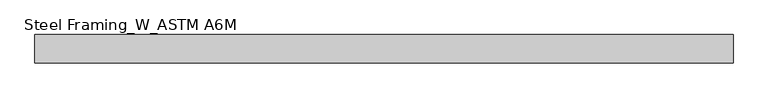
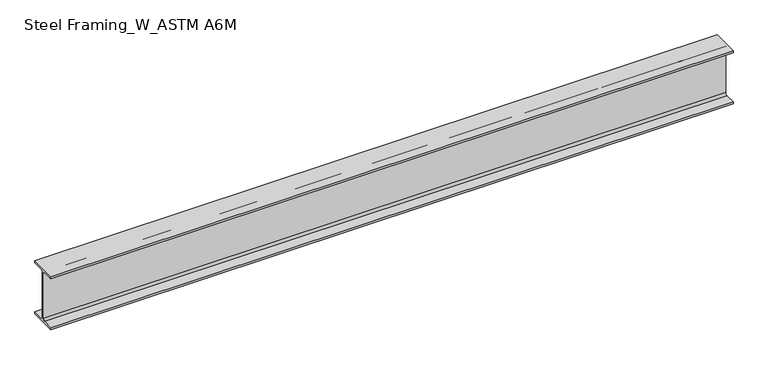
"""IFC4 building model written with IfcOpenShell, lengths in millimetres: beam geometry, Steel Framing_W_ASTM A6M : H_SB_AR_S02_W200x22.5_J1."""

from ifc_helpers import new_model, si_unit, point, frame, frame_2d, origin, place, context, project, spatial, polyline, circle_curve, trimmed, segment, composite_curve, outline, extrude, source, transform, mapped, element, save


def steel_framing_w_astm_a6m_fd7f4403(model_context):
    return source(origin(), model_context, "Body", "SweptSolid", [
        extrude(outline(composite_curve([segment(polyline([(51.0, -95.0), (51.0, -103.0), (-51.0, -103.0), (-51.0, -95.0), (-10.71, -95.0)]), True, "CONTINUOUS"), segment(trimmed(circle_curve(frame_2d((-10.71, -87.4)), 7.6), [point((-10.71, -95.0))], [point((-3.11, -87.4))], True, "CARTESIAN"), True, "CONTINUOUS"), segment(polyline([(-3.11, -87.4), (-3.11, 87.4)]), True, "CONTINUOUS"), segment(trimmed(circle_curve(frame_2d((-10.71, 87.4)), 7.6), [point((-3.11, 87.4))], [point((-10.71, 95.0))], True, "CARTESIAN"), True, "CONTINUOUS"), segment(polyline([(-10.71, 95.0), (-51.0, 95.0), (-51.0, 103.0), (51.0, 103.0), (51.0, 95.0), (10.71, 95.0)]), True, "CONTINUOUS"), segment(trimmed(circle_curve(frame_2d((10.71, 87.4)), 7.6), [point((10.71, 95.0))], [point((3.11, 87.4))], True, "CARTESIAN"), True, "CONTINUOUS"), segment(polyline([(3.11, 87.4), (3.11, -87.4)]), True, "CONTINUOUS"), segment(trimmed(circle_curve(frame_2d((10.71, -87.4)), 7.6), [point((3.11, -87.4))], [point((10.71, -95.0))], True, "CARTESIAN"), True, "CONTINUOUS"), segment(polyline([(10.71, -95.0), (51.0, -95.0)]), True, "CONTINUOUS")], self_intersect=False)), frame((-1252.8, 0.0, 0.0), z_axis=(1.0, 0.0, 0.0), x_axis=(0.0, 1.0, 0.0)), (0.0, 0.0, 1.0), 2505.6),
    ])


if __name__ == "__main__":
    model = new_model("IFC4")
    model_context = context("Model", 3, world=origin())
    ifc_project = project(units=[si_unit("LENGTHUNIT", "METRE", prefix="MILLI")], contexts=[model_context])
    site = spatial("IfcSite", under=ifc_project)
    building = spatial("IfcBuilding", under=site)
    placement = place(None, origin())
    steel_framing_w_astm_a6m_shape = steel_framing_w_astm_a6m_fd7f4403(model_context)
    element("IfcBeam", 1, ObjectType="Steel Framing_W_ASTM A6M : H_SB_AR_S02_W200x22.5_J1", at=placement, inside=building, context=model_context, shape_type="MappedRepresentation", body=[
        mapped(steel_framing_w_astm_a6m_shape, transform((0.0, 0.0, 0.0), x_axis=(1.0, 0.0, 0.0), y_axis=(0.0, 1.0, 0.0), z_axis=(0.0, 0.0, 1.0))),
    ])
    save(model, "model.ifc")

# Revit data of these elements
# Type "Steel Framing_W_ASTM A6M : H_SB_AR_S02_W200x22.5_J1"
#   Section Name Key = "W8x15"
#   Width = 10.2 cm
#   Web Thickness = 0.622 cm
#   Web Fillet = 0.76 cm
#   Warping Constant = 13900.0 cm⁶
#   Torsional Moment of Inertia = 5.70 cm⁴
#   Section Area = 28.6 cm²
#   Plastic Modulus weak axis = 43.8 cm³
#   Plastic Modulus strong axis = 223.0 cm³
#   Perimeter = 0.795 m²/m
#   Nominal Weight = 22.50 kgf/m
#   Moment of Inertia weak axis = 142.00 cm⁴
#   Moment of Inertia strong axis = 2000.00 cm⁴
#   Height = 20.6 cm
#   Flange Thickness = 0.8 cm
#   Elastic Modulus weak axis = 27.9 cm³
#   Elastic Modulus strong axis = 193.0 cm³
#   Centroid Vertical = 10.3 cm
#   Centroid Horizontal = 5.1 cm
#   Length [instance default] = 1500 mm
#   Structural Material [instance default] = Steel, 45-345
#   Bolt Spacing = 0
#   Assembly Code = ""
# Element 1 (IfcBeam, "Steel Framing_W_ASTM A6M : H_SB_AR_S02_W200x22.5_J1")
#   Materials on its faces: "Steel, 45-345"
# Materials
#   "Steel, 45-345": class "Metal", colour RGB 189 187 185, transparency 0, Description = "Steel 345 MPa", Cost = 0
